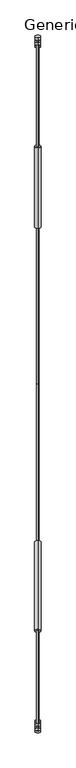
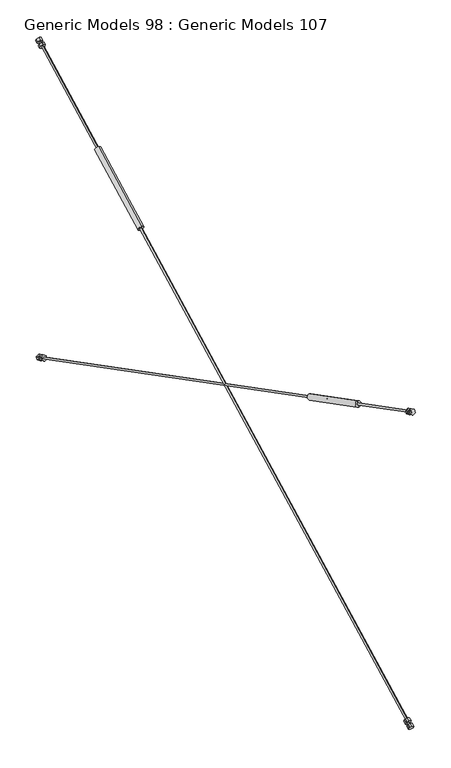
"""IFC4 building model written with IfcOpenShell, lengths in millimetres: proxy geometry, Generic Models 98 : Generic Models 107."""

from ifc_helpers import new_model, si_unit, frame, origin, place, context, project, spatial, polyline, circle_curve, outline, extrude, source, transform, mapped, element, save
from ifc_brep_helpers import plane_surface, cylinder_surface, advanced_brep


def generic_models_98_generic_models_107_f781b15d(model_context):
    return source(origin(), model_context, "Body", "SolidModel", [
        extrude(outline(polyline([(0.0, 0.0), (19.05, 0.0), (28.575, -16.4977839), (19.05, -32.9955679), (0.0, -32.9955679), (-9.525, -16.4977839), (0.0, 0.0)])), frame((31985.9488541, 30937.3190319, 269360.086441), z_axis=(0.0, 0.888197259667458, 0.459462324809356), x_axis=(0.0, 0.459462324809356, -0.888197259667458)), (0.0, 0.0, 1.0), 20.5441692),
        extrude(outline(polyline([(0.0, 0.0), (19.05, 0.0), (28.575, -16.4977839), (19.05, -32.9955679), (0.0, -32.9955679), (-9.525, -16.4977839), (0.0, 0.0)])), frame((31985.9488541, 30905.30865, 269343.5275467), z_axis=(0.0, 0.888197259667458, 0.459462324809356), x_axis=(0.0, 0.459462324809356, -0.888197259667458)), (0.0, 0.0, 1.0), 20.1647216),
        extrude(outline(polyline([(0.0, 0.0), (19.05, 0.0), (28.575, -16.4977839), (19.05, -32.9955679), (0.0, -32.9955679), (-9.525, -16.4977839), (0.0, 0.0)])), frame((31985.9488541, 35146.5791884, 271552.4082287), z_axis=(0.0, 0.888197259667458, 0.459462324809356), x_axis=(0.0, 0.459462324809356, -0.888197259667458)), (0.0, 0.0, 1.0), 19.3390334),
        extrude(outline(polyline([(0.0, 0.0), (19.05, 0.0), (28.575, -16.4977839), (19.05, -32.9955679), (0.0, -32.9955679), (-9.525, -16.4977839), (0.0, 0.0)])), frame((31985.9488541, 35117.5604412, 271537.3969), z_axis=(0.0, 0.888197259667458, 0.459462324809356), x_axis=(0.0, 0.459462324809356, -0.888197259667458)), (0.0, 0.0, 1.0), 16.7965118),
        extrude(outline(polyline([(0.0, 0.0), (19.05, 0.0), (28.575, -16.497784), (19.05, -32.9955679), (0.0, -32.9955679), (-9.525, -16.497784), (0.0, 0.0)])), frame((32018.944422, 35129.7490253, 269365.7757312), z_axis=(0.0, -0.888197259667458, 0.459462324809356), x_axis=(0.0, -0.459462324809356, -0.888197259667458)), (0.0, 0.0, 1.0), 21.4463119),
        extrude(outline(polyline([(0.0, 0.0), (19.05, 0.0), (28.575, -16.497784), (19.05, -32.9955679), (0.0, -32.9955679), (-9.525, -16.497784), (0.0, 0.0)])), frame((32018.944422, 35164.2725821, 269347.918684), z_axis=(0.0, -0.888197259667458, 0.459462324809356), x_axis=(0.0, -0.459462324809356, -0.888197259667458)), (0.0, 0.0, 1.0), 22.9938079),
        extrude(outline(polyline([(0.0, 0.0), (19.05, 0.0), (28.575, -16.497784), (19.05, -32.9955679), (0.0, -32.9955679), (-9.525, -16.497784), (0.0, 0.0)])), frame((32018.944422, 30914.2123618, 271545.8928313), z_axis=(0.0, -0.888197259667458, 0.459462324809356), x_axis=(0.0, -0.459462324809356, -0.888197259667458)), (0.0, 0.0, 1.0), 16.299243),
        extrude(outline(polyline([(0.0, 0.0), (19.05, 0.0), (28.575, -16.497784), (19.05, -32.9955679), (0.0, -32.9955679), (-9.525, -16.497784), (0.0, 0.0)])), frame((32018.944422, 30941.6062211, 271531.7239596), z_axis=(0.0, -0.888197259667458, 0.459462324809356), x_axis=(0.0, -0.459462324809356, -0.888197259667458)), (0.0, 0.0, 1.0), 14.9666526),
        advanced_brep(
        [(32002.446638, 34006.9565579, 270926.8701514), (32002.446638, 33989.3568642, 270960.661582), (32002.446638, 34482.859803, 271217.6942207), (32002.446638, 34500.4594967, 271183.9027901), (32002.446638, 33998.1567111, 270943.7658667), (32002.446638, 34491.6596498, 271200.7985054)],
        [
            (0, 1, circle_curve(frame((32002.446638, 33998.1567111, 270943.7658667), z_axis=(0.0, 0.8869141886573364, 0.461934218215428), x_axis=(0.0, -0.4619342182154281, 0.8869141886573366)), 19.05)),
            (1, 2),
            (2, 3, circle_curve(frame((32002.446638, 34491.6596498, 271200.7985054), z_axis=(0.0, -0.8869141886573364, -0.461934218215428), x_axis=(0.0, -0.4619342182154281, 0.8869141886573366)), 19.05)),
            (3, 0),
            (1, 0, circle_curve(frame((32002.446638, 33998.1567111, 270943.7658667), z_axis=(0.0, 0.8869141886573364, 0.461934218215428), x_axis=(0.0, -0.4619342182154281, 0.8869141886573366)), 19.05)),
            (3, 2, circle_curve(frame((32002.446638, 34491.6596498, 271200.7985054), z_axis=(0.0, -0.8869141886573364, -0.461934218215428), x_axis=(0.0, -0.4619342182154281, 0.8869141886573366)), 19.05)),
            (4, 1),
            (0, 4),
            (2, 5),
            (5, 3),
        ],
        [
            cylinder_surface(frame((32002.446638, 35170.5810798, 271554.4032216), z_axis=(0.0, -0.8869141886573364, -0.461934218215428), x_axis=(0.0, -0.4619342182154281, 0.8869141886573366)), 19.05),
            plane_surface(frame((32002.446638, 33998.1567111, 270943.7658667), z_axis=(0.0, -0.8869141886573364, -0.461934218215428), x_axis=(0.0, -0.461934218215428, 0.8869141886573364))),
            plane_surface(frame((32002.446638, 34491.6596498, 271200.7985054), z_axis=(0.0, 0.8869141886573364, 0.461934218215428), x_axis=(0.0, -0.461934218215428, 0.8869141886573364))),
        ],
        [
            (0, [[1, 2, 3, 4]]),
            (0, [[5, -4, 6, -2]]),
            (1, [[7, -1, 8]]),
            (1, [[-8, -5, -7]]),
            (2, [[-3, 9, 10]]),
            (2, [[-6, -10, -9]]),
        ],
    ),
        advanced_brep(
        [(32002.446638, 34291.352297, 271089.3121613), (32002.446638, 34285.4857324, 271100.5759715), (32002.446638, 35159.5267468, 271555.8054151), (32002.446638, 35165.3933113, 271544.5416049), (32002.446638, 34288.4190147, 271094.9440664), (32002.446638, 35162.4600291, 271550.17351)],
        [
            (0, 1, circle_curve(frame((32002.446638, 34288.4190147, 271094.9440664), z_axis=(0.0, 0.8869141886573364, 0.461934218215428), x_axis=(0.0, -0.4619342182154281, 0.8869141886573366)), 6.35)),
            (1, 2),
            (2, 3, circle_curve(frame((32002.446638, 35162.4600291, 271550.17351), z_axis=(0.0, -0.8869141886573364, -0.461934218215428), x_axis=(0.0, -0.4619342182154281, 0.8869141886573366)), 6.35)),
            (3, 0),
            (1, 0, circle_curve(frame((32002.446638, 34288.4190147, 271094.9440664), z_axis=(0.0, 0.8869141886573364, 0.461934218215428), x_axis=(0.0, -0.4619342182154281, 0.8869141886573366)), 6.35)),
            (3, 2, circle_curve(frame((32002.446638, 35162.4600291, 271550.17351), z_axis=(0.0, -0.8869141886573364, -0.461934218215428), x_axis=(0.0, -0.4619342182154281, 0.8869141886573366)), 6.35)),
            (4, 1),
            (0, 4),
            (2, 5),
            (5, 3),
        ],
        [
            cylinder_surface(frame((32002.446638, 35170.5810798, 271554.4032216), z_axis=(0.0, -0.8869141886573364, -0.461934218215428), x_axis=(0.0, -0.4619342182154281, 0.8869141886573366)), 6.35),
            plane_surface(frame((32002.446638, 34288.4190147, 271094.9440664), z_axis=(0.0, -0.8869141886573364, -0.461934218215428), x_axis=(0.0, -0.461934218215428, 0.8869141886573364))),
            plane_surface(frame((32002.446638, 35162.4600291, 271550.17351), z_axis=(0.0, 0.8869141886573364, 0.461934218215428), x_axis=(0.0, -0.461934218215428, 0.8869141886573364))),
        ],
        [
            (0, [[1, 2, 3, 4]]),
            (0, [[5, -4, 6, -2]]),
            (1, [[7, -1, 8]]),
            (1, [[-8, -5, -7]]),
            (2, [[-3, 9, 10]]),
            (2, [[-6, -10, -9]]),
        ],
    ),
        advanced_brep(
        [(32002.446638, 30917.4542489, 269332.0745648), (32002.446638, 30911.5876844, 269343.338375), (32002.446638, 34178.5949266, 271044.9037075), (32002.446638, 34184.4614911, 271033.6398973), (32002.446638, 30914.5209667, 269337.7064699), (32002.446638, 34181.5282089, 271039.2718024)],
        [
            (0, 1, circle_curve(frame((32002.446638, 30914.5209667, 269337.7064699), z_axis=(0.0, 0.8869141886573364, 0.461934218215428), x_axis=(0.0, -0.4619342182154281, 0.8869141886573366)), 6.35)),
            (1, 2),
            (2, 3, circle_curve(frame((32002.446638, 34181.5282089, 271039.2718024), z_axis=(0.0, -0.8869141886573364, -0.461934218215428), x_axis=(0.0, -0.4619342182154281, 0.8869141886573366)), 6.35)),
            (3, 0),
            (1, 0, circle_curve(frame((32002.446638, 30914.5209667, 269337.7064699), z_axis=(0.0, 0.8869141886573364, 0.461934218215428), x_axis=(0.0, -0.4619342182154281, 0.8869141886573366)), 6.35)),
            (3, 2, circle_curve(frame((32002.446638, 34181.5282089, 271039.2718024), z_axis=(0.0, -0.8869141886573364, -0.461934218215428), x_axis=(0.0, -0.4619342182154281, 0.8869141886573366)), 6.35)),
            (4, 1),
            (0, 4),
            (2, 5),
            (5, 3),
        ],
        [
            cylinder_surface(frame((32002.446638, 35170.5810798, 271554.4032216), z_axis=(0.0, -0.8869141886573364, -0.461934218215428), x_axis=(0.0, -0.4619342182154281, 0.8869141886573366)), 6.35),
            plane_surface(frame((32002.446638, 30914.5209667, 269337.7064699), z_axis=(0.0, -0.8869141886573364, -0.461934218215428), x_axis=(0.0, -0.461934218215428, 0.8869141886573364))),
            plane_surface(frame((32002.446638, 34181.5282089, 271039.2718024), z_axis=(0.0, 0.8869141886573364, 0.461934218215428), x_axis=(0.0, -0.461934218215428, 0.8869141886573364))),
        ],
        [
            (0, [[1, 2, 3, 4]]),
            (0, [[5, -4, 6, -2]]),
            (1, [[7, -1, 8]]),
            (1, [[-8, -5, -7]]),
            (2, [[-3, 9, 10]]),
            (2, [[-6, -10, -9]]),
        ],
    ),
        advanced_brep(
        [(32002.446638, 31514.6763467, 271224.9356439), (32002.446638, 31523.4272991, 271241.8567352), (32002.446638, 31505.9253943, 271208.0145525), (32002.446638, 32069.1104806, 270959.649906), (32002.446638, 32051.6085758, 270925.8077233), (32002.446638, 32060.3595282, 270942.7288146)],
        [
            (0, 1),
            (1, 2, circle_curve(frame((32002.446638, 31514.6763467, 271224.9356439), z_axis=(0.0, -0.888246265022081, 0.45936757904136327), x_axis=(0.0, 0.45936757904136327, 0.888246265022081)), 19.05)),
            (2, 0),
            (2, 1, circle_curve(frame((32002.446638, 31514.6763467, 271224.9356439), z_axis=(0.0, -0.888246265022081, 0.45936757904136327), x_axis=(0.0, 0.45936757904136327, 0.888246265022081)), 19.05)),
            (1, 3),
            (3, 4, circle_curve(frame((32002.446638, 32060.3595282, 270942.7288146), z_axis=(0.0, -0.888246265022081, 0.45936757904136327), x_axis=(0.0, 0.45936757904136327, 0.888246265022081)), 19.05)),
            (4, 2),
            (4, 3, circle_curve(frame((32002.446638, 32060.3595282, 270942.7288146), z_axis=(0.0, -0.888246265022081, 0.45936757904136327), x_axis=(0.0, 0.45936757904136327, 0.888246265022081)), 19.05)),
            (3, 5),
            (5, 4),
        ],
        [
            plane_surface(frame((32002.446638, 31514.6763467, 271224.9356439), z_axis=(0.0, -0.888246265022081, 0.45936757904136327), x_axis=(0.0, 0.45936757904136327, 0.888246265022081))),
            cylinder_surface(frame((32002.446638, 30892.6375966, 271546.6307029), z_axis=(0.0, -0.888246265022081, 0.45936757904136327), x_axis=(0.0, 0.45936757904136327, 0.888246265022081)), 19.05),
            plane_surface(frame((32002.446638, 32060.3595282, 270942.7288146), z_axis=(0.0, 0.888246265022081, -0.45936757904136327), x_axis=(0.0, 0.45936757904136327, 0.888246265022081))),
        ],
        [
            (0, [[1, 2, 3]]),
            (0, [[-3, 4, -1]]),
            (1, [[-2, 5, 6, 7]]),
            (1, [[-4, -7, 8, -5]]),
            (2, [[-6, 9, 10]]),
            (2, [[-8, -10, -9]]),
        ],
    ),
        advanced_brep(
        [(32002.446638, 30896.9278508, 271544.4119447), (32002.446638, 30899.844844, 271550.0523261), (32002.446638, 30894.0108576, 271538.7715634), (32002.446638, 31708.3694443, 271131.9137953), (32002.446638, 31702.5354579, 271120.6330326), (32002.446638, 31705.4524511, 271126.2734139)],
        [
            (0, 1),
            (1, 2, circle_curve(frame((32002.446638, 30896.9278508, 271544.4119447), z_axis=(0.0, -0.888246265022081, 0.45936757904136327), x_axis=(0.0, 0.45936757904136327, 0.888246265022081)), 6.3500198)),
            (2, 0),
            (2, 1, circle_curve(frame((32002.446638, 30896.9278508, 271544.4119447), z_axis=(0.0, -0.888246265022081, 0.45936757904136327), x_axis=(0.0, 0.45936757904136327, 0.888246265022081)), 6.3500198)),
            (1, 3),
            (3, 4, circle_curve(frame((32002.446638, 31705.4524511, 271126.2734139), z_axis=(0.0, -0.888246265022081, 0.45936757904136327), x_axis=(0.0, 0.45936757904136327, 0.888246265022081)), 6.3500198)),
            (4, 2),
            (4, 3, circle_curve(frame((32002.446638, 31705.4524511, 271126.2734139), z_axis=(0.0, -0.888246265022081, 0.45936757904136327), x_axis=(0.0, 0.45936757904136327, 0.888246265022081)), 6.3500198)),
            (3, 5),
            (5, 4),
        ],
        [
            plane_surface(frame((32002.446638, 30896.9278508, 271544.4119447), z_axis=(0.0, -0.888246265022081, 0.45936757904136327), x_axis=(0.0, 0.45936757904136327, 0.888246265022081))),
            cylinder_surface(frame((32002.446638, 30892.6375966, 271546.6307029), z_axis=(0.0, -0.888246265022081, 0.45936757904136327), x_axis=(0.0, 0.45936757904136327, 0.888246265022081)), 6.3500198),
            plane_surface(frame((32002.446638, 31705.4524511, 271126.2734139), z_axis=(0.0, 0.888246265022081, -0.45936757904136327), x_axis=(0.0, 0.45936757904136327, 0.888246265022081))),
        ],
        [
            (0, [[1, 2, 3]]),
            (0, [[-3, 4, -1]]),
            (1, [[-2, 5, 6, 7]]),
            (1, [[-4, -7, 8, -5]]),
            (2, [[-6, 9, 10]]),
            (2, [[-8, -10, -9]]),
        ],
    ),
        advanced_brep(
        [(32002.446638, 31836.4250988, 271058.5392838), (32002.446638, 31839.342092, 271064.1796652), (32002.446638, 31833.5081056, 271052.8989024), (32002.446638, 35161.1532239, 269346.2638149), (32002.446638, 35155.3192375, 269334.9830521), (32002.446638, 35158.2362307, 269340.6234335)],
        [
            (0, 1),
            (1, 2, circle_curve(frame((32002.446638, 31836.4250988, 271058.5392838), z_axis=(0.0, -0.888246265022081, 0.45936757904136327), x_axis=(0.0, 0.45936757904136327, 0.888246265022081)), 6.3500198)),
            (2, 0),
            (2, 1, circle_curve(frame((32002.446638, 31836.4250988, 271058.5392838), z_axis=(0.0, -0.888246265022081, 0.45936757904136327), x_axis=(0.0, 0.45936757904136327, 0.888246265022081)), 6.3500198)),
            (1, 3),
            (3, 4, circle_curve(frame((32002.446638, 35158.2362307, 269340.6234335), z_axis=(0.0, -0.888246265022081, 0.45936757904136327), x_axis=(0.0, 0.45936757904136327, 0.888246265022081)), 6.3500198)),
            (4, 2),
            (4, 3, circle_curve(frame((32002.446638, 35158.2362307, 269340.6234335), z_axis=(0.0, -0.888246265022081, 0.45936757904136327), x_axis=(0.0, 0.45936757904136327, 0.888246265022081)), 6.3500198)),
            (3, 5),
            (5, 4),
        ],
        [
            plane_surface(frame((32002.446638, 31836.4250988, 271058.5392838), z_axis=(0.0, -0.888246265022081, 0.45936757904136327), x_axis=(0.0, 0.45936757904136327, 0.888246265022081))),
            cylinder_surface(frame((32002.446638, 30892.6375966, 271546.6307029), z_axis=(0.0, -0.888246265022081, 0.45936757904136327), x_axis=(0.0, 0.45936757904136327, 0.888246265022081)), 6.3500198),
            plane_surface(frame((32002.446638, 35158.2362307, 269340.6234335), z_axis=(0.0, 0.888246265022081, -0.45936757904136327), x_axis=(0.0, 0.45936757904136327, 0.888246265022081))),
        ],
        [
            (0, [[1, 2, 3]]),
            (0, [[-3, 4, -1]]),
            (1, [[-2, 5, 6, 7]]),
            (1, [[-4, -7, 8, -5]]),
            (2, [[-6, 9, 10]]),
            (2, [[-8, -10, -9]]),
        ],
    ),
    ])


if __name__ == "__main__":
    model = new_model("IFC4")
    model_context = context("Model", 3, world=origin())
    ifc_project = project(units=[si_unit("LENGTHUNIT", "METRE", prefix="MILLI")], contexts=[model_context])
    site = spatial("IfcSite", under=ifc_project)
    building = spatial("IfcBuilding", under=site)
    placement = place(None, origin())
    generic_models_98_generic_models_107_shape = generic_models_98_generic_models_107_f781b15d(model_context)
    element("IfcBuildingElementProxy", 1, Name="Generic Models 98 : Generic Models 107", ObjectType="Generic Models 98 : Generic Models 107", at=placement, inside=building, context=model_context, shape_type="MappedRepresentation", body=[
        mapped(generic_models_98_generic_models_107_shape, transform((0.0, 0.0, 0.0), x_axis=(1.0, 0.0, 0.0), y_axis=(0.0, 1.0, 0.0), z_axis=(0.0, 0.0, 1.0))),
    ])
    save(model, "model.ifc")

# Revit data of these elements
# Element 1 (IfcBuildingElementProxy, "Generic Models 98 : Generic Models 107")
#   Materials on its faces: "1/2\" DIA. GALV. ROD", "TURN BUCKLE"
# Materials
#   "1/2\" DIA. GALV. ROD": class "Metal", colour RGB 199 199 199, transparency 0, Description = "Carbon steel", Cost = 0
#   "TURN BUCKLE": class "Metal", colour RGB 199 199 199, transparency 0, Description = "Carbon steel", Cost = 0
